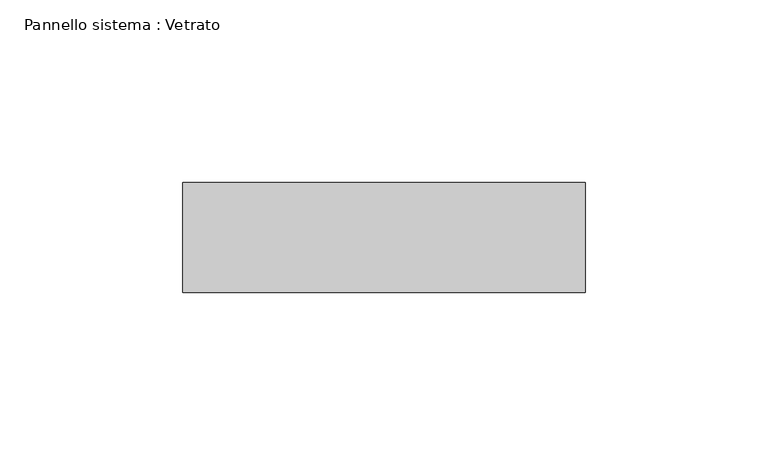
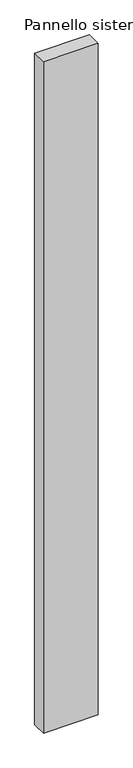
"""IFC4 building model written with IfcOpenShell, lengths in millimetres: plate geometry, Pannello sistema : Vetrato."""

from ifc_helpers import new_model, si_unit, origin, origin_with_axes, place, context, project, spatial, polyline, outline, extrude, source, transform, mapped, element, save


def pannello_sistema_vetrato_3d7c56e5(model_context):
    return source(origin(), model_context, "Body", "SweptSolid", [
        extrude(outline(polyline([(55.0, -15.0), (-55.0, -15.0), (-55.0, 15.0), (55.0, 15.0), (55.0, -15.0)])), origin_with_axes(), (0.0, 0.0, 1.0), 1425.0),
    ])


if __name__ == "__main__":
    model = new_model("IFC4")
    model_context = context("Model", 3, world=origin())
    ifc_project = project(units=[si_unit("LENGTHUNIT", "METRE", prefix="MILLI")], contexts=[model_context])
    site = spatial("IfcSite", under=ifc_project)
    building = spatial("IfcBuilding", under=site)
    placement = place(None, origin())
    pannello_sistema_vetrato_shape = pannello_sistema_vetrato_3d7c56e5(model_context)
    element("IfcPlate", 1, ObjectType="Pannello sistema : Vetrato", at=placement, inside=building, context=model_context, shape_type="MappedRepresentation", body=[
        mapped(pannello_sistema_vetrato_shape, transform((0.0, 0.0, 0.0), x_axis=(1.0, 0.0, 0.0), y_axis=(0.0, 1.0, 0.0), z_axis=(0.0, 0.0, 1.0))),
    ])
    save(model, "model.ifc")

# Revit data of these elements
# Type "Pannello sistema : Vetrato"
#   Construction Type Id = "GSP4R"
#   Analytic Construction = "Vetrata singola Pilkington 1/8 in"
#   Visual Light Transmittance = 0.9
#   Solar Heat Gain Coefficient = 0.86
#   Heat Transfer Coefficient (U) = 6.7069 W/(m²·K)
# Element 1 (IfcPlate, "Pannello sistema : Vetrato")
#   Materials on its faces: "Default - Vetro"
# Materials
#   "Default - Vetro": class "Vetro", colour RGB 208 208 208, transparency 0.7, Cost = 0
